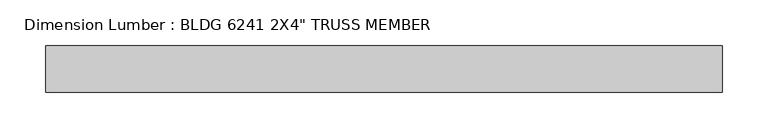
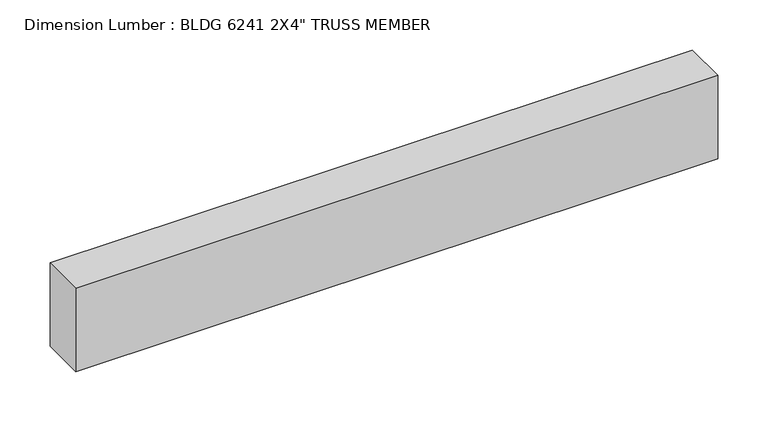
"""IFC4 building model written with IfcOpenShell, lengths in millimetres: beam geometry."""

from ifc_helpers import new_model, si_unit, frame, origin, place, context, project, spatial, polyline, outline, extrude, source, transform, mapped, element, save


def beam_7b112a02(model_context):
    return source(origin(), model_context, "Body", "SweptSolid", [
        extrude(outline(polyline([(371.7582386, 25.4), (371.7582386, -25.4), (-368.3, -25.4), (-368.3, 25.4), (371.7582386, 25.4)])), frame((0.0, 0.0, -50.8), z_axis=(0.0, 0.0, 1.0), x_axis=(1.0, 0.0, 0.0)), (0.0, 0.0, 1.0), 101.6),
    ])


if __name__ == "__main__":
    model = new_model("IFC4")
    model_context = context("Model", 3, world=origin())
    ifc_project = project(units=[si_unit("LENGTHUNIT", "METRE", prefix="MILLI")], contexts=[model_context])
    site = spatial("IfcSite", under=ifc_project)
    building = spatial("IfcBuilding", under=site)
    placement = place(None, origin())
    beam_shape = beam_7b112a02(model_context)
    element("IfcBeam", 1, ObjectType="Dimension Lumber : BLDG 6241 2X4\" TRUSS MEMBER", at=placement, inside=building, context=model_context, shape_type="MappedRepresentation", body=[
        mapped(beam_shape, transform((0.0, 0.0, 0.0), x_axis=(1.0, 0.0, 0.0), y_axis=(0.0, 1.0, 0.0), z_axis=(0.0, 0.0, 1.0))),
    ])
    save(model, "model.ifc")

# Revit data of these elements
# Type "Dimension Lumber : BLDG 6241 2X4\" TRUSS MEMBER"
#   Assembly Code = "B10"
#   A = 0.273472 SF
#   Length [instance default] = 5' - 0"
#   b = 0' - 2"
#   d = 0' - 4"
#   Structural Material [instance default] = Softwood, Lumber
# Element 1 (IfcBeam, "Dimension Lumber : BLDG 6241 2X4\" TRUSS MEMBER")
#   Materials on its faces: "Softwood, Lumber"
# Materials
#   "Softwood, Lumber": class "Wood", colour RGB 223 192 134, transparency 0, Description = "Pinus Echinata", Cost = 0
